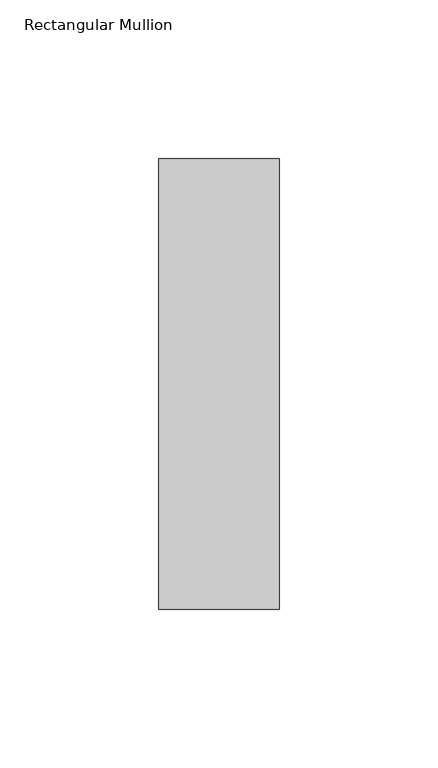
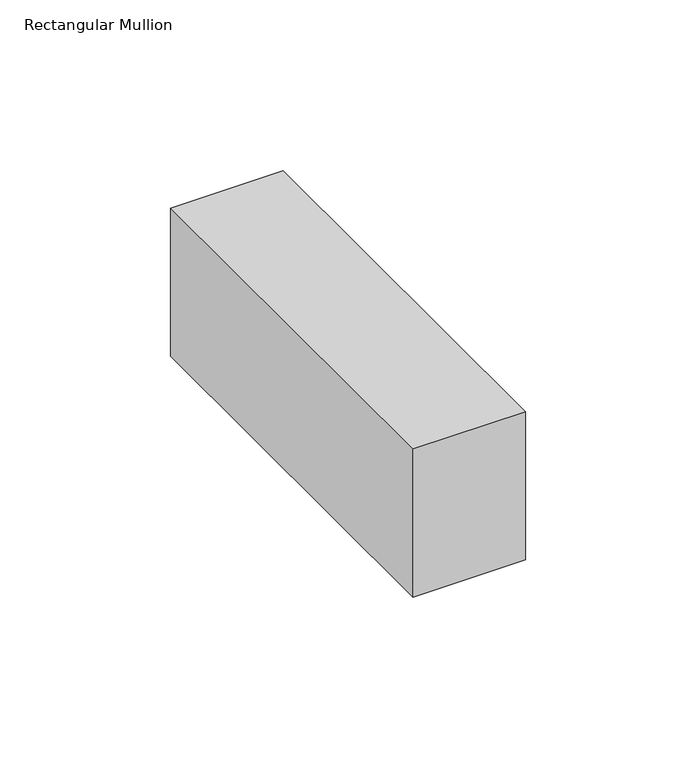
"""IFC4 building model written with IfcOpenShell, lengths in millimetres: member geometry, Rectangular Mullion : NLRS_21_CWM_hsb-regel 38x142_gen_rsf."""

from ifc_helpers import new_model, si_unit, frame, origin, place, context, project, spatial, polyline, outline, extrude, source, transform, mapped, element, save


def rectangular_mullion_7080d8a8(model_context):
    return source(origin(), model_context, "Body", "SweptSolid", [
        extrude(outline(polyline([(-38.0, -71.0), (-38.0, 71.0), (0.0, 71.0), (0.0, -71.0), (-38.0, -71.0)])), frame((0.0, 0.0, -52.9999997), z_axis=(0.0, 0.0, 1.0), x_axis=(1.0, 0.0, 0.0)), (0.0, 0.0, 1.0), 52.9999997),
    ])


if __name__ == "__main__":
    model = new_model("IFC4")
    model_context = context("Model", 3, world=origin())
    ifc_project = project(units=[si_unit("LENGTHUNIT", "METRE", prefix="MILLI")], contexts=[model_context])
    site = spatial("IfcSite", under=ifc_project)
    building = spatial("IfcBuilding", under=site)
    placement = place(None, origin())
    rectangular_mullion_shape = rectangular_mullion_7080d8a8(model_context)
    element("IfcMember", 1, ObjectType="Rectangular Mullion : NLRS_21_CWM_hsb-regel 38x142_gen_rsf", at=placement, inside=building, context=model_context, shape_type="MappedRepresentation", body=[
        mapped(rectangular_mullion_shape, transform((0.0, 0.0, 0.0), x_axis=(1.0, 0.0, 0.0), y_axis=(0.0, 1.0, 0.0), z_axis=(0.0, 0.0, 1.0))),
    ])
    save(model, "model.ifc")

# Revit data of these elements
# Type "Rectangular Mullion : NLRS_21_CWM_hsb-regel 38x142_gen_rsf"
#   Export Type to IFC As = "IfcWall"
#   Type IfcGUID = "07M7mRoiH1CR8m_RSKIwpF"
#   Assembly Code = "21.10"
#   built-in parameter 1007322 = 0.465879 (stored number, unit not read)
#   built-in parameter 1007321 = 0.062336 (stored number, unit not read)
#   built-in parameter 1007320 = 0.062336 (stored number, unit not read)
# Element 1 (IfcMember, "Rectangular Mullion : NLRS_21_CWM_hsb-regel 38x142_gen_rsf")
#   Materials on its faces: "NLRS_i2_hout naaldhout vuren_gen_rsf"
# Materials
#   "NLRS_i2_hout naaldhout vuren_gen_rsf": class "I - Hout", colour RGB 234 199 147, transparency 0, Keynote = "i2", Manufacturer = "Revit Standards Foundation", URL = "www.revitstandards.org", Description = "hout vuren", Cost = 0
